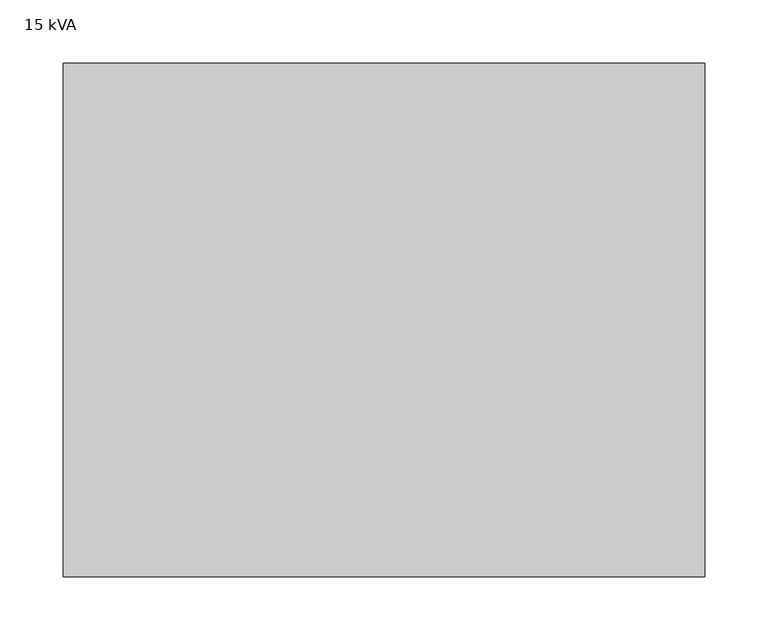
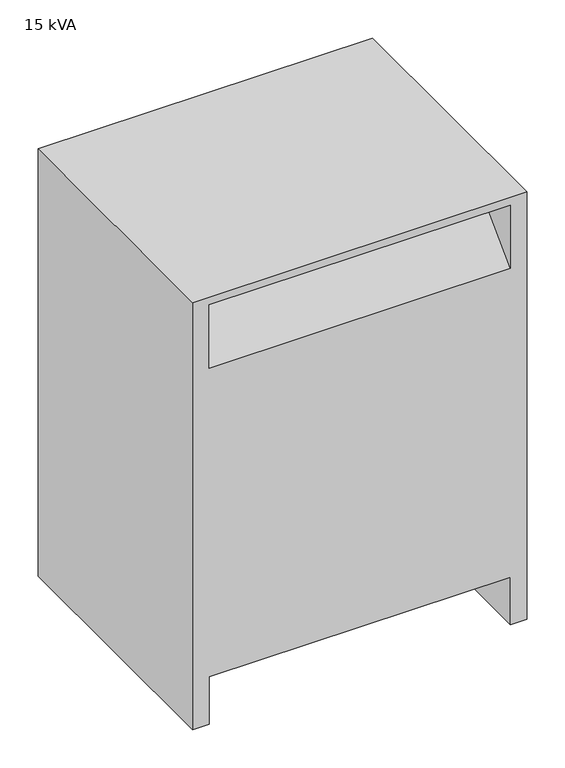
"""IFC4 building model written with IfcOpenShell, lengths in millimetres: proxy geometry, Dry Type Transformer - 480-208Y120 - NEMA Type 2 : 15 kVA."""

from ifc_helpers import new_model, si_unit, origin, place, context, project, spatial, faceted_brep, source, transform, mapped, element, save


def proxy_15_kva_b0f935c8(model_context):
    return source(origin(), model_context, "Body", "Brep", [
        faceted_brep([(254.0, -21.6841349, 685.8), (254.0, 384.7158651, 685.8), (-254.0, 384.7158651, 685.8), (-254.0, -21.6841349, 685.8), (-254.0, -21.6841349, 0.0), (-254.0, 384.7158651, 0.0), (-228.6, 384.7158651, 0.0), (-228.6, -21.6841349, 0.0), (254.0, 384.7158651, 0.0), (254.0, -21.6841349, 0.0), (228.6, -21.6841349, 0.0), (228.6, 384.7158651, 0.0), (228.6, 384.7158651, 76.2), (-228.6, 384.7158651, 76.2), (228.6, 384.7158651, 571.5), (228.6, 384.7158651, 673.1), (-228.6, 384.7158651, 673.1), (-228.6, 384.7158651, 571.5), (-228.6, -21.6841349, 76.2), (228.6, -21.6841349, 76.2), (228.6, -21.6841349, 673.1), (228.6, -21.6841349, 571.5), (-228.6, -21.6841349, 571.5), (-228.6, -21.6841349, 673.1), (228.6, 79.9158651, 673.1), (-228.6, 79.9158651, 673.1), (228.6, 283.1158651, 673.1), (-228.6, 283.1158651, 673.1)], [[[0, 1, 2, 3]], [[4, 5, 6, 7]], [[8, 9, 10, 11]], [[1, 0, 9, 8]], [[2, 1, 8, 11, 12, 13, 6, 5], [14, 15, 16, 17]], [[3, 2, 5, 4]], [[0, 3, 4, 7, 18, 19, 10, 9], [20, 21, 22, 23]], [[18, 13, 12, 19]], [[13, 18, 7, 6]], [[19, 12, 11, 10]], [[24, 21, 20]], [[25, 23, 22]], [[24, 20, 23, 25]], [[21, 24, 25, 22]], [[26, 15, 14]], [[27, 17, 16]], [[26, 14, 17, 27]], [[15, 26, 27, 16]]]),
    ])


if __name__ == "__main__":
    model = new_model("IFC4")
    model_context = context("Model", 3, world=origin())
    ifc_project = project(units=[si_unit("LENGTHUNIT", "METRE", prefix="MILLI")], contexts=[model_context])
    site = spatial("IfcSite", under=ifc_project)
    building = spatial("IfcBuilding", under=site)
    placement = place(None, origin())
    proxy_15_kva_shape = proxy_15_kva_b0f935c8(model_context)
    element("IfcBuildingElementProxy", 1, Name="Dry Type Transformer - 480-208Y120 - NEMA Type 2 : 15 kVA", ObjectType="Dry Type Transformer - 480-208Y120 - NEMA Type 2 : 15 kVA", at=placement, inside=building, context=model_context, shape_type="MappedRepresentation", body=[
        mapped(proxy_15_kva_shape, transform((0.0, 0.0, 0.0), x_axis=(1.0, 0.0, 0.0), y_axis=(0.0, 1.0, 0.0), z_axis=(0.0, 0.0, 1.0))),
    ])
    save(model, "model.ifc")

# Revit data of these elements
# Type "Dry Type Transformer - 480-208Y120 - NEMA Type 2 : 15 kVA"
#   built-in parameter 1140083 [instance default] = "Type 2"
#   Transformer Length = 1' - 8"
#   Primary Voltage = 480 V
#   Transformer Height = 2' - 3"
#   built-in parameter 1140140 [instance default] = 1 (stored number, unit not read)
#   Transformer Width = 1' - 4"
#   built-in parameter 1140142 [instance default] = -1
#   Primary Number of Poles = 3
#   built-in parameter 1140079 [instance default] = 3
#   Transformer Material = none
#   Load Classification = Transformer
#   Default Elevation = 0
#   Assembly Code = ""
#   built-in parameter 1140087 [instance default] = 1
